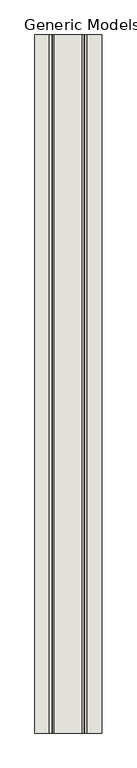
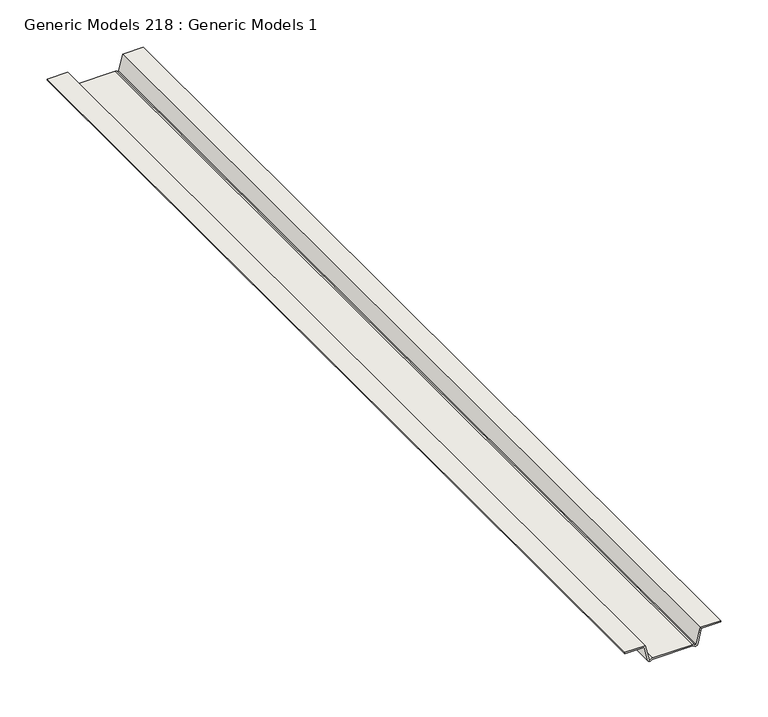
"""IFC4 building model written with IfcOpenShell, lengths in millimetres: wall geometry, Generic Models 218 : Generic Models 1."""

import ifcopenshell
import ifcopenshell.guid

model = None  # the IFC model being written
_history = None  # IfcOwnerHistory: only IFC2X3 demands one
_inside = {}  # id of a spatial element -> (the spatial element, [elements in it])
_under = {}  # id of a project, library or spatial element -> (it, [spatial elements below it])
_declared = {}  # id of a project -> (the project, [libraries it declares])
_typed = {}  # id of a type object -> (the type object, [elements of that type])
_made_of = {}  # id of a material, layer set ... -> (it, [elements and type objects made of it])


def new_model(schema):
    """Start an empty IFC model of exactly this schema.

    Asked for "IFC4X3", IfcOpenShell would pick the latest addendum, in which some entities
    have other attributes; the version numbers below select the first issue.
    IFC2X3 requires an IfcOwnerHistory on every rooted entity: one is made here for all.
    """
    global model, _history
    if schema == "IFC4X3":
        model = ifcopenshell.file(schema_version=(4, 3, 0, 0))
    else:
        model = ifcopenshell.file(schema=schema)
    _inside.clear()
    _under.clear()
    _declared.clear()
    _typed.clear()
    _made_of.clear()
    _history = None
    if model.schema == "IFC2X3":
        org = make("IfcOrganization", Name="unknown")
        user = make(
            "IfcPersonAndOrganization",
            ThePerson=make("IfcPerson", FamilyName="unknown"),
            TheOrganization=org,
        )
        app = make(
            "IfcApplication",
            ApplicationDeveloper=org,
            Version="unknown",
            ApplicationFullName="unknown",
            ApplicationIdentifier="unknown",
        )
        _history = make(
            "IfcOwnerHistory",
            OwningUser=user,
            OwningApplication=app,
            ChangeAction="ADDED",
            CreationDate=0,
        )
    return model


def make(cls, **values):
    """One entity of the class cls with the attributes given. An attribute that is None is left unset."""
    return model.create_entity(
        cls, **{name: value for name, value in values.items() if value is not None}
    )


def rooted(cls, **values):
    """An entity with a GlobalId (a new one), such as an element, a storey or a relation."""
    return make(cls, GlobalId=ifcopenshell.guid.new(), OwnerHistory=_history, **values)


def si_unit(unit_type, name, prefix=None):
    """IfcSIUnit, for example si_unit("LENGTHUNIT", "METRE", prefix="MILLI")."""
    return make("IfcSIUnit", UnitType=unit_type, Prefix=prefix, Name=name)


def assignment(units):
    """IfcUnitAssignment: the units of a project."""
    return None if units is None else make("IfcUnitAssignment", Units=units)


def point(xyz):
    """IfcCartesianPoint."""
    return None if xyz is None else make("IfcCartesianPoint", Coordinates=xyz)


def direction(xyz):
    """IfcDirection."""
    return None if xyz is None else make("IfcDirection", DirectionRatios=xyz)


def frame(location, z_axis=None, x_axis=None):
    """IfcAxis2Placement3D, a coordinate frame: its origin and axes. An axis left out is left unset."""
    return make(
        "IfcAxis2Placement3D",
        Location=point(location),
        Axis=direction(z_axis),
        RefDirection=direction(x_axis),
    )


def frame_2d(location, x_axis=None):
    """IfcAxis2Placement2D, a coordinate frame in the plane: its origin and x axis."""
    return make(
        "IfcAxis2Placement2D", Location=point(location), RefDirection=direction(x_axis)
    )


def origin():
    """The frame at (0, 0, 0) with its axes left unset."""
    return frame((0.0, 0.0, 0.0))


def place(relative_to, where):
    """IfcLocalPlacement: puts the frame where relative to a parent placement (None: the world)."""
    return make(
        "IfcLocalPlacement", PlacementRelTo=relative_to, RelativePlacement=where
    )


def context(
    kind, dimensions, precision=None, world=None, true_north=None, identifier=None
):
    """IfcGeometricRepresentationContext, for example the 3D "Model" context."""
    return make(
        "IfcGeometricRepresentationContext",
        ContextIdentifier=identifier,
        ContextType=kind,
        CoordinateSpaceDimension=dimensions,
        Precision=precision,
        WorldCoordinateSystem=world,
        TrueNorth=true_north,
    )


def project(units=None, contexts=None):
    """IfcProject with its units and contexts."""
    return rooted(
        "IfcProject",
        Name="project",
        RepresentationContexts=contexts,
        UnitsInContext=assignment(units),
    )


def spatial(cls, under=None, at=None, **own):
    """A site, building, storey or space (cls), placed at a placement, below another one or the project."""
    s = rooted(cls, ObjectPlacement=at, **own)
    if under is not None:
        _under.setdefault(under.id(), (under, []))[1].append(s)
    return s


def polyline(points):
    """IfcPolyline through the points."""
    return make("IfcPolyline", Points=[point(p) for p in points])


def circle_curve(where, radius):
    """IfcCircle in the frame where."""
    return make("IfcCircle", Position=where, Radius=radius)


def trimmed(basis, trim1, trim2, sense, master):
    """IfcTrimmedCurve: the piece of a basis curve between two trims."""
    return make(
        "IfcTrimmedCurve",
        BasisCurve=basis,
        Trim1=trim1,
        Trim2=trim2,
        SenseAgreement=sense,
        MasterRepresentation=master,
    )


def segment(curve, same_sense, transition):
    """IfcCompositeCurveSegment."""
    return make(
        "IfcCompositeCurveSegment",
        Transition=transition,
        SameSense=same_sense,
        ParentCurve=curve,
    )


def composite_curve(segments, self_intersect=None):
    """IfcCompositeCurve: segments joined end to end."""
    return make("IfcCompositeCurve", Segments=segments, SelfIntersect=self_intersect)


def outline(outer, holes=None, kind="AREA"):
    """IfcArbitraryClosedProfileDef: a profile drawn as a closed curve; with holes, ...WithVoids."""
    if holes is None:
        return make("IfcArbitraryClosedProfileDef", ProfileType=kind, OuterCurve=outer)
    return make(
        "IfcArbitraryProfileDefWithVoids",
        ProfileType=kind,
        OuterCurve=outer,
        InnerCurves=holes,
    )


def extrude(swept, where, along, depth):
    """IfcExtrudedAreaSolid: the profile swept, set in the frame where, extruded along a direction by depth."""
    return make(
        "IfcExtrudedAreaSolid",
        SweptArea=swept,
        Position=where,
        ExtrudedDirection=direction(along),
        Depth=depth,
    )


def shape(context_of_items, identifier, shape_type, items):
    """IfcShapeRepresentation: the items that make up one representation, for example the "Body"."""
    return make(
        "IfcShapeRepresentation",
        ContextOfItems=context_of_items,
        RepresentationIdentifier=identifier,
        RepresentationType=shape_type,
        Items=items,
    )


def source(mapping_origin, context_of_items, identifier, shape_type, items):
    """IfcRepresentationMap: a shape defined once, which mapped items show again and again."""
    return make(
        "IfcRepresentationMap",
        MappingOrigin=mapping_origin,
        MappedRepresentation=shape(context_of_items, identifier, shape_type, items),
    )


def transform(
    local_origin,
    x_axis=None,
    y_axis=None,
    z_axis=None,
    scale=None,
    scale2=None,
    scale3=None,
    uniform=True,
):
    """IfcCartesianTransformationOperator3D, or its non-uniform kind. x_axis, y_axis, z_axis: its Axis1, 2, 3."""
    if uniform:
        return make(
            "IfcCartesianTransformationOperator3D",
            Axis1=direction(x_axis),
            Axis2=direction(y_axis),
            LocalOrigin=point(local_origin),
            Scale=scale,
            Axis3=direction(z_axis),
        )
    return make(
        "IfcCartesianTransformationOperator3DnonUniform",
        Axis1=direction(x_axis),
        Axis2=direction(y_axis),
        LocalOrigin=point(local_origin),
        Scale=scale,
        Axis3=direction(z_axis),
        Scale2=scale2,
        Scale3=scale3,
    )


def mapped(mapping_source, mapping_target):
    """IfcMappedItem: shows the shape of a source again, moved by a transform."""
    return make(
        "IfcMappedItem", MappingSource=mapping_source, MappingTarget=mapping_target
    )


def made_of(thing, what):
    """Note that an element or type object is made of a material, layer set ...; save() writes the relation."""
    if what is not None:
        _made_of.setdefault(what.id(), (what, []))[1].append(thing)
    return thing


def element(
    cls,
    number,
    at=None,
    inside=None,
    cuts=None,
    type_object=None,
    material=None,
    context=None,
    identifier="Body",
    shape_type=None,
    held_by="IfcProductDefinitionShape",
    body=None,
    shapes=None,
    **own,
):
    """One element of the class cls, such as IfcWall. Its Tag is "e" and its number.

    at: its placement. inside: the storey or other place that contains it. cuts: it is an
    opening in that element (IfcRelVoidsElement). A single representation is given by context,
    identifier, shape_type and body (its items); several are given by shapes. held_by: the class
    of the entity that holds the representations. save() writes the other relations.
    """
    e = rooted(cls, Tag="e%d" % number, ObjectPlacement=at, **own)
    if body is not None:
        shapes = [shape(context, identifier, shape_type, body)]
    if shapes is not None:
        e.Representation = make(held_by, Representations=shapes)
    if inside is not None:
        _inside.setdefault(inside.id(), (inside, []))[1].append(e)
    if cuts is not None:
        rooted(
            "IfcRelVoidsElement", RelatingBuildingElement=cuts, RelatedOpeningElement=e
        )
    if type_object is not None:
        _typed.setdefault(type_object.id(), (type_object, []))[1].append(e)
    return made_of(e, material)


def aggregate(whole, parts):
    """IfcRelAggregates: a whole, such as a stair, and the parts it consists of."""
    return rooted("IfcRelAggregates", RelatingObject=whole, RelatedObjects=parts)


def save(model, path):
    """Write the relations noted so far, then the file.

    IfcRelAggregates (storeys below a building ...), IfcRelContainedInSpatialStructure (elements
    in a storey), IfcRelDefinesByType, IfcRelAssociatesMaterial and IfcRelDeclares: one each for
    every whole, place, type object, material and project.
    """
    for whole, parts in _under.values():
        aggregate(whole, parts)
    for where, things in _inside.values():
        rooted(
            "IfcRelContainedInSpatialStructure",
            RelatedElements=things,
            RelatingStructure=where,
        )
    for kind, things in _typed.values():
        rooted("IfcRelDefinesByType", RelatedObjects=things, RelatingType=kind)
    for what, things in _made_of.values():
        rooted("IfcRelAssociatesMaterial", RelatedObjects=things, RelatingMaterial=what)
    for by, libraries in _declared.values():
        rooted("IfcRelDeclares", RelatingContext=by, RelatedDefinitions=libraries)
    model.write(path)


def generic_models_218_generic_models_1_b9d2597b(model_context):
    return source(origin(), model_context, "Body", "SweptSolid", [
        extrude(outline(composite_curve([segment(polyline([(2079.7402211, 398014.3223812), (2079.7402211, 398038.1009707), (2081.3277211, 398038.1009707), (2081.3277211, 398013.0468669), (2061.3130097, 398008.6323984)]), True, "CONTINUOUS"), segment(trimmed(circle_curve(frame_2d((2061.4839711, 398007.8572783)), 0.79375), [point((2061.3130097, 398008.6323984))], [point((2060.9548045, 398007.2656519))], True, "CARTESIAN"), True, "CONTINUOUS"), segment(trimmed(circle_curve(frame_2d((2058.3089711, 398004.3075203)), 3.96875), [point((2060.9548045, 398007.2656519))], [point((2062.2777211, 398004.3075203))], False, "CARTESIAN"), True, "CONTINUOUS"), segment(polyline([(2062.2777211, 398004.3075203), (2062.2777211, 397955.2189784)]), True, "CONTINUOUS"), segment(trimmed(circle_curve(frame_2d((2058.3089711, 397955.2189784)), 3.96875), [point((2062.2777211, 397955.2189784))], [point((2060.9548045, 397952.2608468))], False, "CARTESIAN"), True, "CONTINUOUS"), segment(trimmed(circle_curve(frame_2d((2061.4839711, 397951.6692205)), 0.79375), [point((2060.9548045, 397952.2608468))], [point((2061.3130097, 397950.8941003))], True, "CARTESIAN"), True, "CONTINUOUS"), segment(polyline([(2061.3130097, 397950.8941003), (2081.3277211, 397946.4796318), (2081.3277211, 397921.425528), (2079.7402211, 397921.425528), (2079.7402211, 397945.2041175), (2060.9710869, 397949.34386)]), True, "CONTINUOUS"), segment(trimmed(circle_curve(frame_2d((2061.4839711, 397951.6692205)), 2.38125), [point((2060.9710869, 397949.34386))], [point((2059.8964711, 397953.4440994))], False, "CARTESIAN"), True, "CONTINUOUS"), segment(trimmed(circle_curve(frame_2d((2058.3089711, 397955.2189784)), 2.38125), [point((2059.8964711, 397953.4440994))], [point((2060.6902211, 397955.2189784))], True, "CARTESIAN"), True, "CONTINUOUS"), segment(polyline([(2060.6902211, 397955.2189784), (2060.6902211, 398004.3075203)]), True, "CONTINUOUS"), segment(trimmed(circle_curve(frame_2d((2058.3089711, 398004.3075203)), 2.38125), [point((2060.6902211, 398004.3075203))], [point((2059.8964711, 398006.0823993))], True, "CARTESIAN"), True, "CONTINUOUS"), segment(trimmed(circle_curve(frame_2d((2061.4839711, 398007.8572783)), 2.38125), [point((2059.8964711, 398006.0823993))], [point((2060.9710869, 398010.1826387))], False, "CARTESIAN"), True, "CONTINUOUS"), segment(polyline([(2060.9710869, 398010.1826387), (2079.7402211, 398014.3223812)]), True, "CONTINUOUS")], self_intersect=False)), frame((0.0, 0.0, 0.0), z_axis=(0.0, 1.0, 0.0), x_axis=(0.0, 0.0, 1.0)), (0.0, 0.0, 1.0), 1219.2),
    ])


if __name__ == "__main__":
    model = new_model("IFC4")
    model_context = context("Model", 3, world=origin())
    ifc_project = project(units=[si_unit("LENGTHUNIT", "METRE", prefix="MILLI")], contexts=[model_context])
    site = spatial("IfcSite", under=ifc_project)
    building = spatial("IfcBuilding", under=site)
    placement = place(None, origin())
    generic_models_218_generic_models_1_shape = generic_models_218_generic_models_1_b9d2597b(model_context)
    element("IfcWall", 1, ObjectType="Generic Models 218 : Generic Models 1", at=placement, inside=building, context=model_context, shape_type="MappedRepresentation", body=[
        mapped(generic_models_218_generic_models_1_shape, transform((0.0, 0.0, 0.0), x_axis=(1.0, 0.0, 0.0), y_axis=(0.0, 1.0, 0.0), z_axis=(0.0, 0.0, 1.0))),
    ])
    save(model, "model.ifc")

# Revit data of these elements
# Element 1 (IfcWall, "Generic Models 218 : Generic Models 1")
#   Materials on its faces: "7/8\" FURRING CHANNELS @ 12\" O.C."
# Materials
#   "7/8\" FURRING CHANNELS @ 12\" O.C.": class "Unassigned", colour RGB 166 164 162, transparency 0, Keynote = "M05121300.02", Cost = 0
